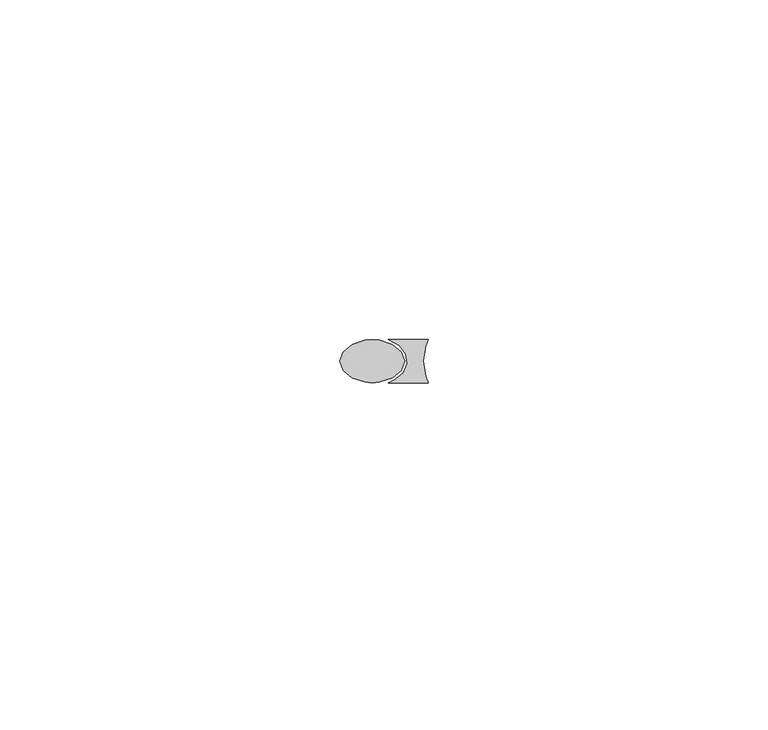
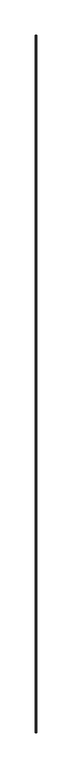
"""IFC4 building model written with IfcOpenShell, lengths in millimetres: proxy geometry, Generic Models 11:Generic Models 1:306267:Generic Models 1:306267 : Generic Models 11:Generic Models 1:306267:300405:Generic Models 1:306267:Generic Models 1:306267 : Generic Models 11:Generic Models 1:306267:300405 : Generic Models 11:Generic Models 1:306267:Generic Models 1:306267 : Generic Models 11:Generic Models 1:306267:300405:16 : Generic Models 11:Generic Models 1:306267:Generic Models 1:306267 : Generic Models 11:Generic Models 1:306267:300405:Generic Models 1:306267:Generic Models 1:306267 : Generic Models 11:Generic Models 1:306267:300405 : Generic Models 11:Generic Models 1:306267:Generic Models 1:306267 : Generic Models 11:Generic Models 1:306267:300405:300182."""

from ifc_helpers import new_model, si_unit, origin, origin_with_axes, place, context, project, spatial, polyline, outline, extrude, source, transform, mapped, element, save


def generic_models_0e2d3967(model_context):
    return source(origin(), model_context, "Body", "SweptSolid", [
        extrude(outline(polyline([(573367.5409469, -536525.0496088), (573366.2194528, -536526.1543429), (573364.3098386, -536526.7674241), (573363.2500826, -536526.8470279), (573362.1903267, -536526.7674241), (573360.2807125, -536526.1543429), (573358.9592184, -536525.0496088), (573358.4875826, -536523.6720279), (573358.9592184, -536522.2944471), (573360.2807125, -536521.189713), (573362.1903267, -536520.5766318), (573363.2500826, -536520.4970279), (573364.3098386, -536520.5766318), (573366.2194528, -536521.189713), (573367.5409469, -536522.2944471), (573368.0125826, -536523.6720279), (573367.5409469, -536525.0496088)])), origin_with_axes(), (0.0, 0.0, 1.0), 6064.4581746),
        extrude(outline(polyline([(573371.1043937, -536521.4627912), (573370.7907076, -536523.6720279), (573371.1043937, -536525.8812647), (573371.4818023, -536526.8470279), (573365.6137102, -536526.8470279), (573366.4739912, -536526.4607104), (573367.7835663, -536525.3772249), (573368.3839199, -536524.0269772), (573368.181132, -536522.6212009), (573367.206927, -536521.3798168), (573365.6137102, -536520.4970279), (573371.4818023, -536520.4970279), (573371.1043937, -536521.4627912)])), origin_with_axes(), (0.0, 0.0, 1.0), 6062.9878028),
    ])


if __name__ == "__main__":
    model = new_model("IFC4")
    model_context = context("Model", 3, world=origin())
    ifc_project = project(units=[si_unit("LENGTHUNIT", "METRE", prefix="MILLI")], contexts=[model_context])
    site = spatial("IfcSite", under=ifc_project)
    building = spatial("IfcBuilding", under=site)
    placement = place(None, origin())
    generic_models_shape = generic_models_0e2d3967(model_context)
    element("IfcBuildingElementProxy", 1, Name="Generic Models 11:Generic Models 1:306267:Generic Models 1:306267 : Generic Models 11:Generic Models 1:306267:300405:Generic Models 1:306267:Generic Models 1:306267 : Generic Models 11:Generic Models 1:306267:300405 : Generic Models 11:Generic Models 1:306267:Generic Models 1:306267 : Generic Models 11:Generic Models 1:306267:300405:16 : Generic Models 11:Generic Models 1:306267:Generic Models 1:306267 : Generic Models 11:Generic Models 1:306267:300405:Generic Models 1:306267:Generic Models 1:306267 : Generic Models 11:Generic Models 1:306267:300405 : Generic Models 11:Generic Models 1:306267:Generic Models 1:306267 : Generic Models 11:Generic Models 1:306267:300405:300182", ObjectType="Generic Models 11:Generic Models 1:306267:Generic Models 1:306267 : Generic Models 11:Generic Models 1:306267:300405:Generic Models 1:306267:Generic Models 1:306267 : Generic Models 11:Generic Models 1:306267:300405 : Generic Models 11:Generic Models 1:306267:Generic Models 1:306267 : Generic Models 11:Generic Models 1:306267:300405:16 : Generic Models 11:Generic Models 1:306267:Generic Models 1:306267 : Generic Models 11:Generic Models 1:306267:300405:Generic Models 1:306267:Generic Models 1:306267 : Generic Models 11:Generic Models 1:306267:300405 : Generic Models 11:Generic Models 1:306267:Generic Models 1:306267 : Generic Models 11:Generic Models 1:306267:300405:300182", at=placement, inside=building, context=model_context, shape_type="MappedRepresentation", body=[
        mapped(generic_models_shape, transform((0.0, 0.0, 0.0), x_axis=(1.0, 0.0, 0.0), y_axis=(0.0, 1.0, 0.0), z_axis=(0.0, 0.0, 1.0))),
    ])
    save(model, "model.ifc")

# Revit data of these elements
# Type "Generic Models 11:Generic Models 1:306267:Generic Models 1:306267 : Generic Models 11:Generic Models 1:306267:300405:Generic Models 1:306267:Generic Models 1:306267 : Generic Models 11:Generic Models 1:306267:300405 : Generic Models 11:Generic Models 1:306267:Generic Models 1:306267 : Generic Models 11:Generic Models 1:306267:300405:16 : Generic Models 11:Generic Models 1:306267:Generic Models 1:306267 : Generic Models 11:Generic Models 1:306267:300405:Generic Models 1:306267:Generic Models 1:306267 : Generic Models 11:Generic Models 1:306267:300405 : Generic Models 11:Generic Models 1:306267:Generic Models 1:306267 : Generic Models 11:Generic Models 1:306267:300405:300182"
#   NameOverride = "Generic Models 11:Generic Models 1:306267:Generic Models 1:306267 : Generic Models 11:Generic Models 1:306267:300405:Generic Models 1:306267:Generic Models 1:306267 : Generic Models 11:Generic Models 1:306267:300405 : Generic Models 11:Generic Models 1:306267:Generic Models 1:306267 : Generic Models 11:Generic Models 1:306267:300405:300182"
#   ObjectTypeOverride = "Generic Models 1:306267:Generic Models 1:306267 : Generic Models 11:Generic Models 1:306267:300405 : Generic Models 11:Generic Models 1:306267:Generic Models 1:306267 : Generic Models 11:Generic Models 1:306267:300405"
#   Reference = "Generic Models 1"
#   Tag = "300182"
# Element 1 (IfcBuildingElementProxy, "Generic Models 11:Generic Models 1:306267:Generic Models 1:306267 : Generic Models 11:Generic Models 1:306267:300405:Generic Models 1:306267:Generic Models 1:306267 : Generic Models 11:Generic Models 1:306267:300405 : Generic Models 11:Generic Models 1:306267:Generic Models 1:306267 : Generic Models 11:Generic Models 1:306267:300405:16 : Generic Models 11:Generic Models 1:306267:Generic Models 1:306267 : Generic Models 11:Generic Models 1:306267:300405:Generic Models 1:306267:Generic Models 1:306267 : Generic Models 11:Generic Models 1:306267:300405 : Generic Models 11:Generic Models 1:306267:Generic Models 1:306267 : Generic Models 11:Generic Models 1:306267:300405:300182")
#   Materials on its faces: "SEALANT & BACKER ROD, IF NECESSARY"
# Materials
#   "SEALANT & BACKER ROD, IF NECESSARY": class "Unassigned", colour RGB 120 120 120, transparency 0, Cost = 0
